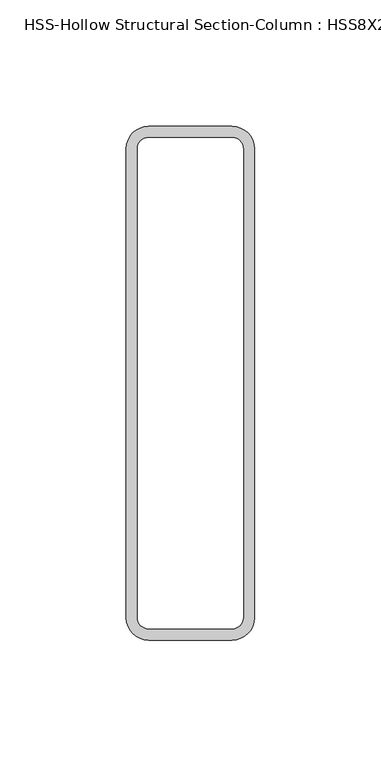
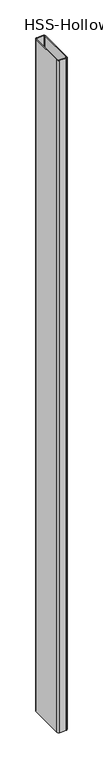
"""IFC4 building model written with IfcOpenShell, lengths in millimetres: column geometry, HSS-Hollow Structural Section-Column : HSS8X2X3/16."""

from ifc_helpers import new_model, si_unit, point, frame, frame_2d, origin, place, context, project, spatial, polyline, circle_curve, trimmed, segment, composite_curve, outline, extrude, source, transform, mapped, element, save


def hss_hollow_structural_section_column_hss8x2x3_16_13fa7c93(model_context):
    return source(origin(), model_context, "Body", "SweptSolid", [
        extrude(outline(composite_curve([segment(trimmed(circle_curve(frame_2d((16.5608, 92.7608)), 8.8392), [point((16.5608, 101.6))], [point((25.4, 92.7608))], False, "CARTESIAN"), True, "CONTINUOUS"), segment(polyline([(25.4, 92.7608), (25.4, -92.7608)]), True, "CONTINUOUS"), segment(trimmed(circle_curve(frame_2d((16.5608, -92.7608)), 8.8392), [point((25.4, -92.7608))], [point((16.5608, -101.6))], False, "CARTESIAN"), True, "CONTINUOUS"), segment(polyline([(16.5608, -101.6), (-16.5608, -101.6)]), True, "CONTINUOUS"), segment(trimmed(circle_curve(frame_2d((-16.5608, -92.7608)), 8.8392), [point((-16.5608, -101.6))], [point((-25.4, -92.7608))], False, "CARTESIAN"), True, "CONTINUOUS"), segment(polyline([(-25.4, -92.7608), (-25.4, 92.7608)]), True, "CONTINUOUS"), segment(trimmed(circle_curve(frame_2d((-16.5608, 92.7608)), 8.8392), [point((-25.4, 92.7608))], [point((-16.5608, 101.6))], False, "CARTESIAN"), True, "CONTINUOUS"), segment(polyline([(-16.5608, 101.6), (16.5608, 101.6)]), True, "CONTINUOUS")], self_intersect=False), holes=[composite_curve([segment(polyline([(16.5608, 97.1804), (-16.5608, 97.1804)]), True, "CONTINUOUS"), segment(trimmed(circle_curve(frame_2d((-16.5608, 92.7608)), 4.4196), [point((-16.5608, 97.1804))], [point((-20.9804, 92.7608))], True, "CARTESIAN"), True, "CONTINUOUS"), segment(polyline([(-20.9804, 92.7608), (-20.9804, -92.7608)]), True, "CONTINUOUS"), segment(trimmed(circle_curve(frame_2d((-16.5608, -92.7608)), 4.4196), [point((-20.9804, -92.7608))], [point((-16.5608, -97.1804))], True, "CARTESIAN"), True, "CONTINUOUS"), segment(polyline([(-16.5608, -97.1804), (16.5608, -97.1804)]), True, "CONTINUOUS"), segment(trimmed(circle_curve(frame_2d((16.5608, -92.7608)), 4.4196), [point((16.5608, -97.1804))], [point((20.9804, -92.7608))], True, "CARTESIAN"), True, "CONTINUOUS"), segment(polyline([(20.9804, -92.7608), (20.9804, 92.7608)]), True, "CONTINUOUS"), segment(trimmed(circle_curve(frame_2d((16.5608, 92.7608)), 4.4196), [point((20.9804, 92.7608))], [point((16.5608, 97.1804))], True, "CARTESIAN"), True, "CONTINUOUS")], self_intersect=False)]), frame((0.0, 0.0, -1200.0), z_axis=(0.0, 0.0, 1.0), x_axis=(1.0, 0.0, 0.0)), (0.0, 0.0, 1.0), 3639.0),
    ])


if __name__ == "__main__":
    model = new_model("IFC4")
    model_context = context("Model", 3, world=origin())
    ifc_project = project(units=[si_unit("LENGTHUNIT", "METRE", prefix="MILLI")], contexts=[model_context])
    site = spatial("IfcSite", under=ifc_project)
    building = spatial("IfcBuilding", under=site)
    placement = place(None, origin())
    hss_hollow_structural_section_column_hss8x2x3_16_shape = hss_hollow_structural_section_column_hss8x2x3_16_13fa7c93(model_context)
    element("IfcColumn", 1, ObjectType="HSS-Hollow Structural Section-Column : HSS8X2X3/16", at=placement, inside=building, context=model_context, shape_type="MappedRepresentation", body=[
        mapped(hss_hollow_structural_section_column_hss8x2x3_16_shape, transform((0.0, 0.0, 0.0), x_axis=(1.0, 0.0, 0.0), y_axis=(0.0, 1.0, 0.0), z_axis=(0.0, 0.0, 1.0))),
    ])
    save(model, "model.ifc")

# Revit data of these elements
# Type "HSS-Hollow Structural Section-Column : HSS8X2X3/16"
#   Assembly Code = "B10"
#   Shape = "Rect."
#   Cost = 1
#   W = 12
#   Ht = 203.2 mm
#   b = 50.8 mm
#   kr = 8.839 mm
#   t = 4.42 mm
#   A = 0.00211612 m²
#   Structural Material [instance default] = Steel ASTM A500, Grade B, Rectangular and Square
# Element 1 (IfcColumn, "HSS-Hollow Structural Section-Column : HSS8X2X3/16")
#   Structural Material = Metal - Steel 43-275
#   Materials on its faces: "Metal - Steel 43-275"
# Materials
#   "Steel ASTM A500, Grade B, Rectangular and Square": class "Metal", colour RGB 199 199 199, transparency 0, Description = "Carbon steel", Cost = 0
#   "Metal - Steel 43-275": class "Metal", colour RGB 247 247 247, transparency 0, Cost = 0
